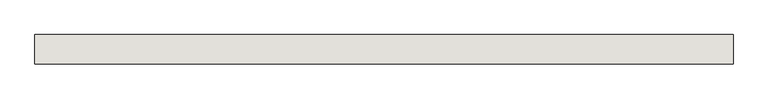
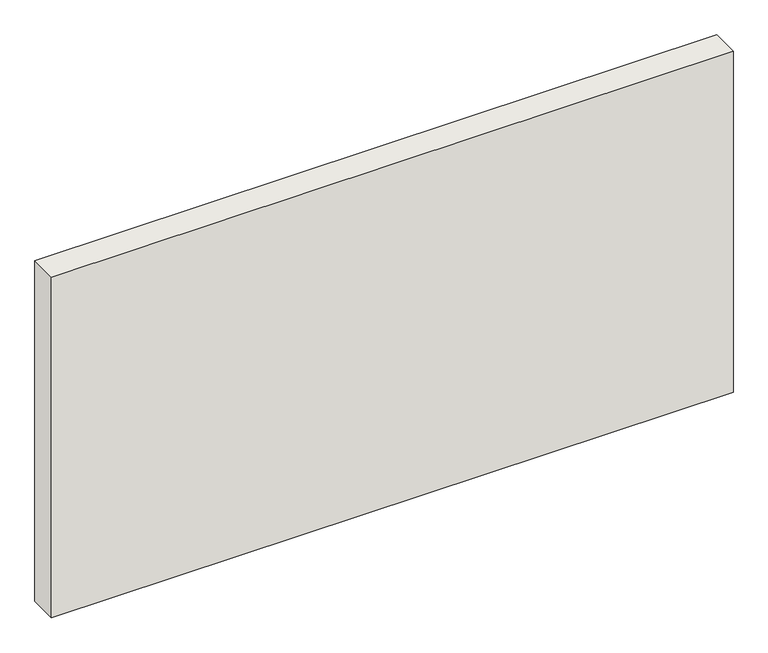
"""IFC4 building model written with IfcOpenShell, lengths in millimetres: wall geometry, Holzwand."""

from ifc_helpers import new_model, si_unit, origin, origin_with_axes, place, context, project, spatial, polyline, outline, extrude, source, transform, mapped, element, save


def wall_b1b9b24f(model_context):
    return source(origin(), model_context, "Body", "SweptSolid", [
        extrude(outline(polyline([(0.0, 200.0), (4750.0, 200.0), (4750.0, 0.0), (0.0, 0.0), (0.0, 200.0)])), origin_with_axes(), (0.0, 0.0, 1.0), 2510.0),
    ])


if __name__ == "__main__":
    model = new_model("IFC4")
    model_context = context("Model", 3, world=origin())
    ifc_project = project(units=[si_unit("LENGTHUNIT", "METRE", prefix="MILLI")], contexts=[model_context])
    site = spatial("IfcSite", under=ifc_project)
    building = spatial("IfcBuilding", under=site)
    placement = place(None, origin())
    wall_shape = wall_b1b9b24f(model_context)
    element("IfcWall", 1, ObjectType="Holzwand", at=placement, inside=building, context=model_context, shape_type="MappedRepresentation", body=[
        mapped(wall_shape, transform((0.0, 0.0, 0.0), x_axis=(1.0, 0.0, 0.0), y_axis=(0.0, 1.0, 0.0), z_axis=(0.0, 0.0, 1.0))),
    ])
    save(model, "model.ifc")

# Revit data of these elements
# Element 1 (IfcWall, "Holzwand")
#   Materials on its faces: "holzschalung"
# Materials
#   "holzschalung": class "Unassigned", colour RGB 128 128 128, transparency 0
